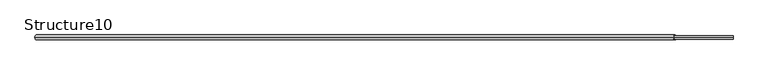
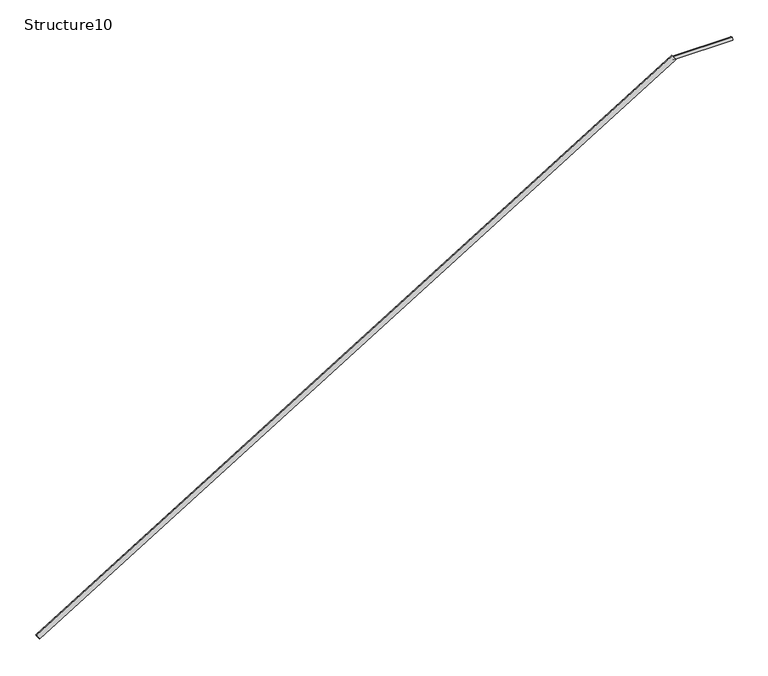
"""IFC4 building model written with IfcOpenShell, lengths in millimetres: proxy geometry, Structure10 : Structure668217131."""

from ifc_helpers import new_model, si_unit, point, frame, frame_2d, origin, place, context, project, spatial, circle_curve, trimmed, segment, composite_curve, outline, extrude, source, transform, mapped, element, save


def structure10_6454dafb(model_context):
    return source(origin(), model_context, "Body", "SweptSolid", [
        extrude(outline(composite_curve([segment(trimmed(circle_curve(frame_2d((1853.7779231, 40961.5078846)), 12.7), [point((1853.7779231, 40948.8078846))], [point((1853.7779231, 40974.2078846))], False, "CARTESIAN"), True, "CONTINUOUS"), segment(trimmed(circle_curve(frame_2d((1853.7779231, 40961.5078846)), 12.7), [point((1853.7779231, 40974.2078846))], [point((1853.7779231, 40948.8078846))], False, "CARTESIAN"), True, "CONTINUOUS")], self_intersect=False)), frame((9816.5238328, 0.0, 0.0), z_axis=(1.0, 0.0, 0.0), x_axis=(0.0, 1.0, 0.0)), (0.0, 0.0, 1.0), 451.286302),
        extrude(outline(composite_curve([segment(trimmed(circle_curve(frame_2d((0.0, -19.05)), 19.05), [point((0.0, -38.1))], [point((0.0, 0.0))], False, "CARTESIAN"), True, "CONTINUOUS"), segment(trimmed(circle_curve(frame_2d((0.0, -19.05)), 19.05), [point((0.0, 0.0))], [point((0.0, -38.1))], False, "CARTESIAN"), True, "CONTINUOUS")], self_intersect=False)), frame((4938.7530423, 1853.7779231, 37988.4648998), z_axis=(0.8523227286500448, 0.0, 0.5230162198503429), x_axis=(0.0, 1.0, 0.0)), (0.0, 0.0, 1.0), 5719.1500287),
    ])


if __name__ == "__main__":
    model = new_model("IFC4")
    model_context = context("Model", 3, world=origin())
    ifc_project = project(units=[si_unit("LENGTHUNIT", "METRE", prefix="MILLI")], contexts=[model_context])
    site = spatial("IfcSite", under=ifc_project)
    building = spatial("IfcBuilding", under=site)
    placement = place(None, origin())
    structure10_shape = structure10_6454dafb(model_context)
    element("IfcBuildingElementProxy", 1, Name="Structure10 : Structure668217131", ObjectType="Structure10 : Structure668217131", at=placement, inside=building, context=model_context, shape_type="MappedRepresentation", body=[
        mapped(structure10_shape, transform((0.0, 0.0, 0.0), x_axis=(1.0, 0.0, 0.0), y_axis=(0.0, 1.0, 0.0), z_axis=(0.0, 0.0, 1.0))),
    ])
    save(model, "model.ifc")

# Revit data of these elements
# Type "Structure10 : Structure668217131"
#   NameOverride = "Structure668217131"
# Element 1 (IfcBuildingElementProxy, "Structure10 : Structure668217131")
#   Materials on its faces: "1.5\" DIA. STAINLESS STEEL RAILING"
# Materials
#   "1.5\" DIA. STAINLESS STEEL RAILING": class "Unassigned", colour RGB 128 128 128, transparency 0, Cost = 0
